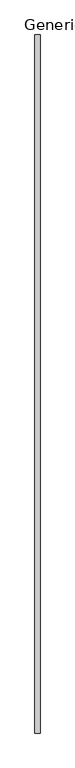
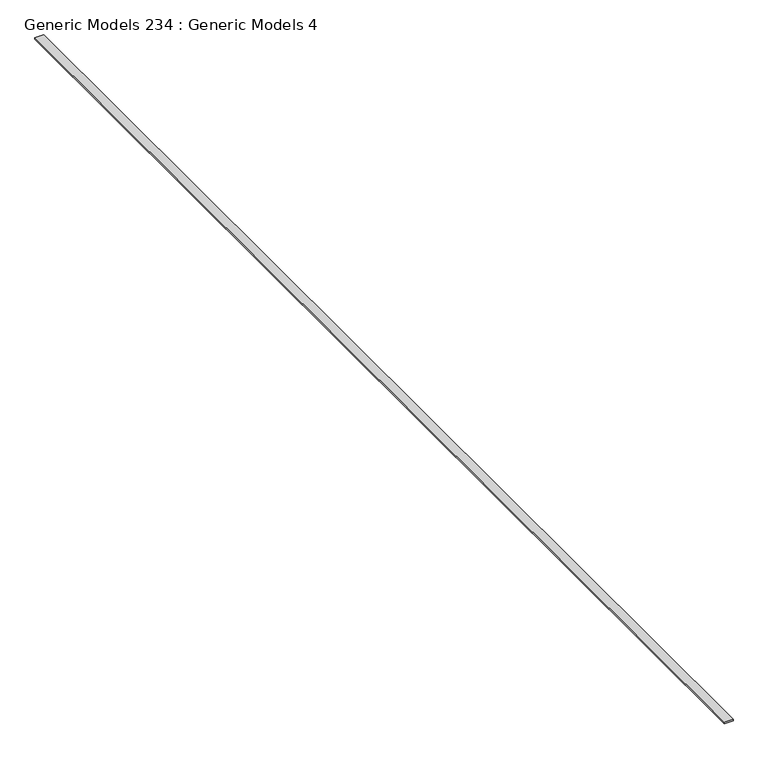
"""IFC4 building model written with IfcOpenShell, lengths in millimetres: proxy geometry, Generic Models 234 : Generic Models 4."""

from ifc_helpers import new_model, si_unit, frame, origin, place, context, project, spatial, polyline, outline, extrude, source, transform, mapped, element, save


def generic_models_234_generic_models_4_5076cbfc(model_context):
    return source(origin(), model_context, "Body", "SweptSolid", [
        extrude(outline(polyline([(36650.8284762, 12775.6158826), (36753.2635788, 12775.6158826), (36753.2635788, -1143.5841174), (36650.8284762, -1143.5841174), (36650.8284762, 12775.6158826)])), frame((0.0, 0.0, 129277.2366834), z_axis=(0.0, 0.0, 1.0), x_axis=(1.0, 0.0, 0.0)), (0.0, 0.0, 1.0), 18.3199747),
    ])


if __name__ == "__main__":
    model = new_model("IFC4")
    model_context = context("Model", 3, world=origin())
    ifc_project = project(units=[si_unit("LENGTHUNIT", "METRE", prefix="MILLI")], contexts=[model_context])
    site = spatial("IfcSite", under=ifc_project)
    building = spatial("IfcBuilding", under=site)
    placement = place(None, origin())
    generic_models_234_generic_models_4_shape = generic_models_234_generic_models_4_5076cbfc(model_context)
    element("IfcBuildingElementProxy", 1, Name="Generic Models 234 : Generic Models 4", ObjectType="Generic Models 234 : Generic Models 4", at=placement, inside=building, context=model_context, shape_type="MappedRepresentation", body=[
        mapped(generic_models_234_generic_models_4_shape, transform((0.0, 0.0, 0.0), x_axis=(1.0, 0.0, 0.0), y_axis=(0.0, 1.0, 0.0), z_axis=(0.0, 0.0, 1.0))),
    ])
    save(model, "model.ifc")

# Revit data of these elements
# Element 1 (IfcBuildingElementProxy, "Generic Models 234 : Generic Models 4")
#   Materials on its faces: "_2X BLOCKING AS REQUIRED"
# Materials
#   "_2X BLOCKING AS REQUIRED": class "Generic", colour RGB 177 130 114, transparency 0, Cost = 0
